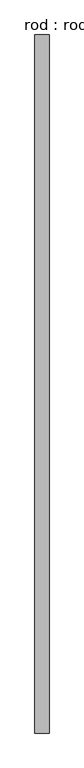
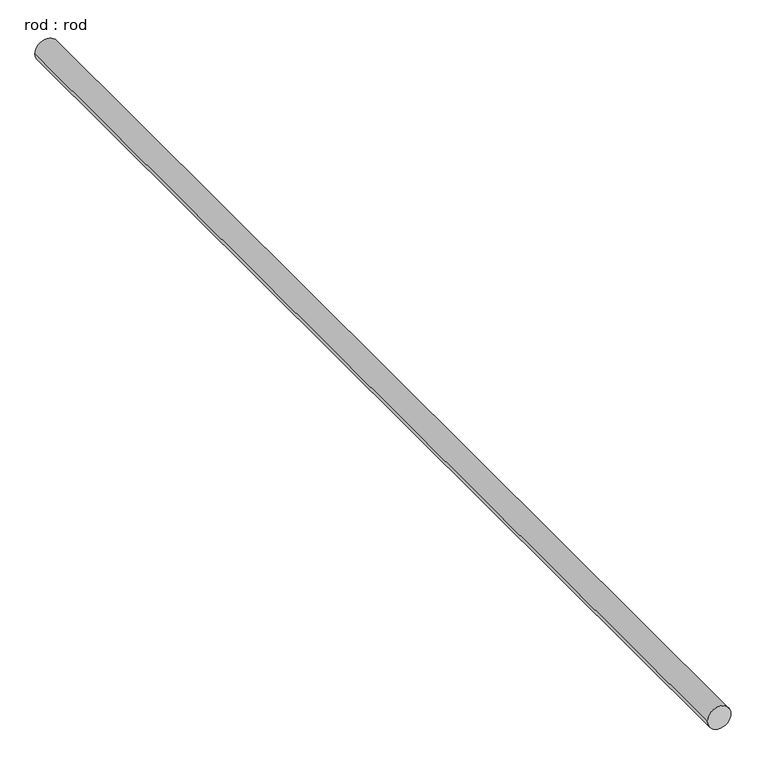
"""IFC4 building model written with IfcOpenShell, lengths in millimetres: proxy geometry, rod : rod."""

from ifc_helpers import new_model, si_unit, point, frame, frame_2d, origin, place, context, project, spatial, circle_curve, trimmed, segment, composite_curve, outline, extrude, source, transform, mapped, element, save


def rod_rod_3f781ba7(model_context):
    return source(origin(), model_context, "Body", "SweptSolid", [
        extrude(outline(composite_curve([segment(trimmed(circle_curve(frame_2d((0.0108462, 0.0)), 200.0), [point((0.0108462, 200.0))], [point((0.0108462, -200.0))], False, "CARTESIAN"), True, "CONTINUOUS"), segment(trimmed(circle_curve(frame_2d((0.0108462, 0.0)), 200.0), [point((0.0108462, -200.0))], [point((0.0108462, 200.0))], False, "CARTESIAN"), True, "CONTINUOUS")], self_intersect=False)), frame((0.0, -5762.0647932, 0.0), z_axis=(0.0, 1.0, 0.0), x_axis=(0.0, 0.0, 1.0)), (0.0, 0.0, 1.0), 19709.5868171),
    ])


if __name__ == "__main__":
    model = new_model("IFC4")
    model_context = context("Model", 3, world=origin())
    ifc_project = project(units=[si_unit("LENGTHUNIT", "METRE", prefix="MILLI")], contexts=[model_context])
    site = spatial("IfcSite", under=ifc_project)
    building = spatial("IfcBuilding", under=site)
    placement = place(None, origin())
    rod_rod_shape = rod_rod_3f781ba7(model_context)
    element("IfcBuildingElementProxy", 1, Name="rod : rod", ObjectType="rod : rod", at=placement, inside=building, context=model_context, shape_type="MappedRepresentation", body=[
        mapped(rod_rod_shape, transform((0.0, 0.0, 0.0), x_axis=(1.0, 0.0, 0.0), y_axis=(0.0, 1.0, 0.0), z_axis=(0.0, 0.0, 1.0))),
    ])
    save(model, "model.ifc")

# Revit data of these elements
# Type "rod : rod"
#   Default Elevation = 0
